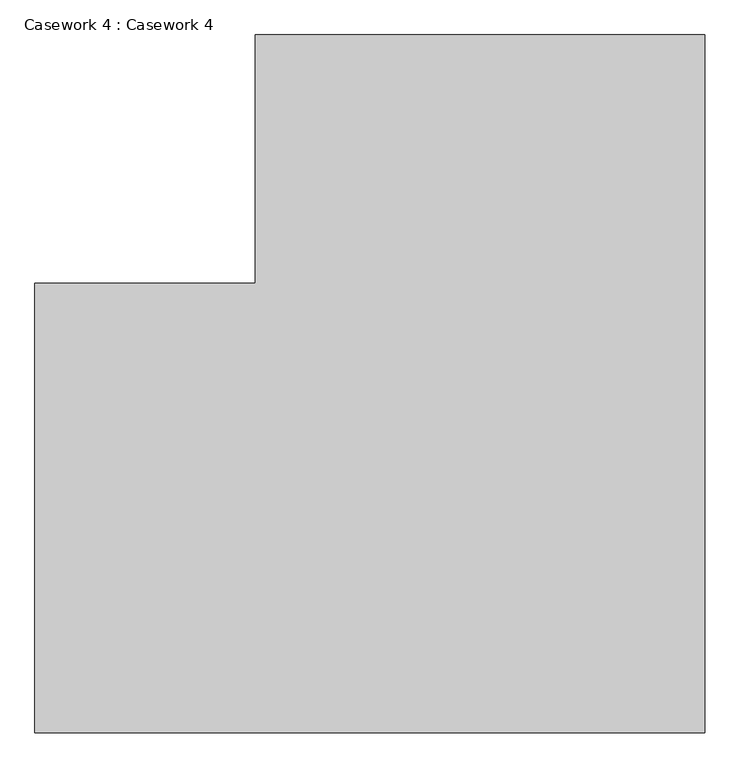
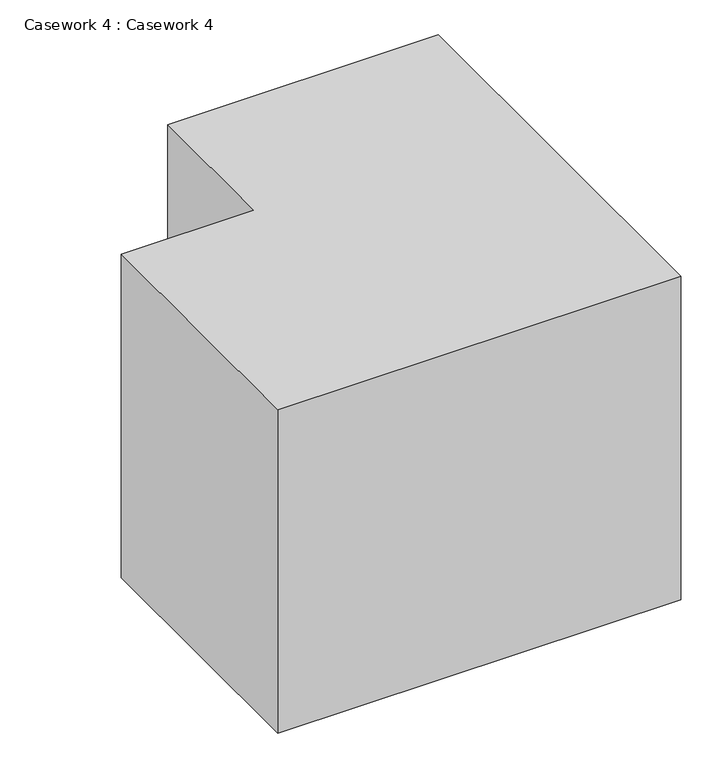
"""IFC4 building model written with IfcOpenShell, lengths in millimetres: furniture geometry, Casework 4 : Casework 4."""

from ifc_helpers import new_model, si_unit, origin, origin_with_axes, place, context, project, spatial, polyline, outline, extrude, source, transform, mapped, element, save


def casework_4_casework_4_6522c02b(model_context):
    return source(origin(), model_context, "Body", "SweptSolid", [
        extrude(outline(polyline([(-44696.5676606, 248427.7599557), (-46134.4732793, 248427.7599557), (-46134.4732793, 249392.9599557), (-45661.7676606, 249392.9599557), (-45661.7676606, 249926.3599557), (-44696.5676606, 249926.3599557), (-44696.5676606, 248427.7599557)])), origin_with_axes(), (0.0, 0.0, 1.0), 1219.2),
    ])


if __name__ == "__main__":
    model = new_model("IFC4")
    model_context = context("Model", 3, world=origin())
    ifc_project = project(units=[si_unit("LENGTHUNIT", "METRE", prefix="MILLI")], contexts=[model_context])
    site = spatial("IfcSite", under=ifc_project)
    building = spatial("IfcBuilding", under=site)
    placement = place(None, origin())
    casework_4_casework_4_shape = casework_4_casework_4_6522c02b(model_context)
    element("IfcFurniture", 1, ObjectType="Casework 4 : Casework 4", at=placement, inside=building, context=model_context, shape_type="MappedRepresentation", body=[
        mapped(casework_4_casework_4_shape, transform((0.0, 0.0, 0.0), x_axis=(1.0, 0.0, 0.0), y_axis=(0.0, 1.0, 0.0), z_axis=(0.0, 0.0, 1.0))),
    ])
    save(model, "model.ifc")

# Revit data of these elements
# Element 1 (IfcFurniture, "Casework 4 : Casework 4")
#   Materials on its faces: "COMPARTMENT SINK WITH SIDE TABLE"
# Materials
#   "COMPARTMENT SINK WITH SIDE TABLE": class "Generic", colour RGB 187 187 187, transparency 0, Cost = 0
